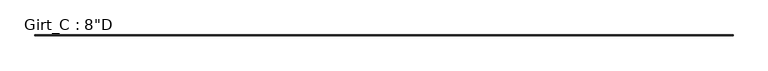
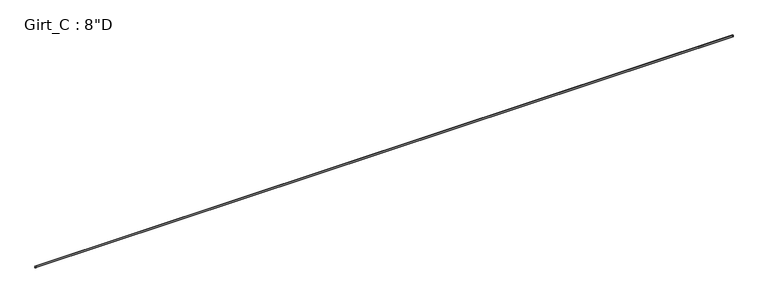
"""IFC4 building model written with IfcOpenShell, lengths in millimetres: beam geometry."""

from ifc_helpers import new_model, si_unit, point, frame, frame_2d, origin, place, context, project, spatial, polyline, circle_curve, trimmed, segment, composite_curve, outline, extrude, source, transform, mapped, element, save


def beam_899dc338(model_context):
    return source(origin(), model_context, "Body", "SweptSolid", [
        extrude(outline(composite_curve([segment(polyline([(87.5109375, 101.6), (99.7560415, 87.0068534), (97.6278742, 85.221109), (86.2154765, 98.821875), (3.3005807, 98.821875)]), True, "CONTINUOUS"), segment(trimmed(circle_curve(frame_2d((3.3741066, 96.8381931)), 1.9850441), [point((3.3005807, 98.821875))], [point((1.3890625, 96.8381931))], True, "CARTESIAN"), True, "CONTINUOUS"), segment(polyline([(1.3890625, 96.8381931), (1.3890625, -96.8389339)]), True, "CONTINUOUS"), segment(trimmed(circle_curve(frame_2d((3.3748024, -96.8389339)), 1.9857399), [point((1.3890625, -96.8389339))], [point((3.2694106, -98.821875))], True, "CARTESIAN"), True, "CONTINUOUS"), segment(polyline([(3.2694106, -98.821875), (86.2154765, -98.821875), (97.6510975, -85.1934327), (99.7792647, -86.979177), (87.5109375, -101.6), (3.3734375, -101.6)]), True, "CONTINUOUS"), segment(trimmed(circle_curve(frame_2d((3.3734375, -96.8375)), 4.7625), [point((3.3734375, -101.6))], [point((-1.3890625, -96.8375))], False, "CARTESIAN"), True, "CONTINUOUS"), segment(polyline([(-1.3890625, -96.8375), (-1.3890625, 96.8375)]), True, "CONTINUOUS"), segment(trimmed(circle_curve(frame_2d((3.3734375, 96.8375)), 4.7625), [point((-1.3890625, 96.8375))], [point((3.3734375, 101.6))], False, "CARTESIAN"), True, "CONTINUOUS"), segment(polyline([(3.3734375, 101.6), (87.5109375, 101.6)]), True, "CONTINUOUS")], self_intersect=False)), frame((-44229.734375, 0.0, 0.0), z_axis=(1.0, 0.0, 0.0), x_axis=(0.0, 1.0, 0.0)), (0.0, 0.0, 1.0), 88284.05),
    ])


if __name__ == "__main__":
    model = new_model("IFC4")
    model_context = context("Model", 3, world=origin())
    ifc_project = project(units=[si_unit("LENGTHUNIT", "METRE", prefix="MILLI")], contexts=[model_context])
    site = spatial("IfcSite", under=ifc_project)
    building = spatial("IfcBuilding", under=site)
    placement = place(None, origin())
    beam_shape = beam_899dc338(model_context)
    element("IfcBeam", 1, ObjectType="Girt_C : 8\"D", at=placement, inside=building, context=model_context, shape_type="MappedRepresentation", body=[
        mapped(beam_shape, transform((0.0, 0.0, 0.0), x_axis=(1.0, 0.0, 0.0), y_axis=(0.0, 1.0, 0.0), z_axis=(0.0, 0.0, 1.0))),
    ])
    save(model, "model.ifc")

# Revit data of these elements
# Type "Girt_C : 8\"D"
#   half leg = 0' - 1 3/4"
#   Web_Thickness = 0' - 0 7/64"
#   Length [instance default] = 10' - 0"
#   Leg_1 = 0' - 3 1/2"
#   Height = 0' - 8"
#   Structural Material [instance default] = none
# Element 1 (IfcBeam, "Girt_C : 8\"D")
#   Structural Material = CEE' SECTION (8.0x3.5C - SEE STRUCT. DWGS)
#   Materials on its faces: "CEE' SECTION (8.0x3.5C - SEE STRUCT. DWGS)"
# Materials
#   "CEE' SECTION (8.0x3.5C - SEE STRUCT. DWGS)": class "Metal", colour RGB 137 146 153, transparency 0, Description = "Steel, mill finish", Cost = 0
